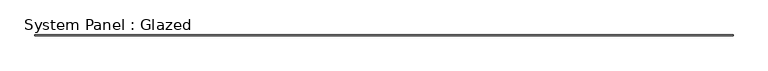
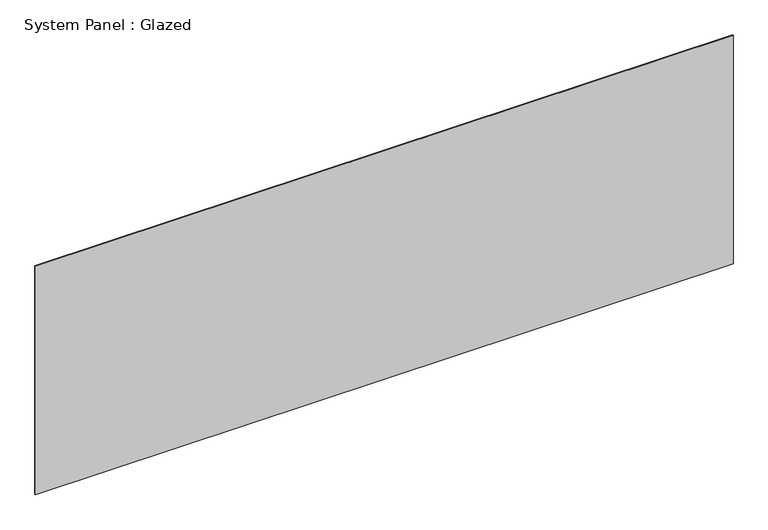
"""IFC4 building model written with IfcOpenShell, lengths in millimetres: plate geometry, System Panel : Glazed."""

import ifcopenshell
import ifcopenshell.guid

model = None  # the IFC model being written
_history = None  # IfcOwnerHistory: only IFC2X3 demands one
_inside = {}  # id of a spatial element -> (the spatial element, [elements in it])
_under = {}  # id of a project, library or spatial element -> (it, [spatial elements below it])
_declared = {}  # id of a project -> (the project, [libraries it declares])
_typed = {}  # id of a type object -> (the type object, [elements of that type])
_made_of = {}  # id of a material, layer set ... -> (it, [elements and type objects made of it])


def new_model(schema):
    """Start an empty IFC model of exactly this schema.

    Asked for "IFC4X3", IfcOpenShell would pick the latest addendum, in which some entities
    have other attributes; the version numbers below select the first issue.
    IFC2X3 requires an IfcOwnerHistory on every rooted entity: one is made here for all.
    """
    global model, _history
    if schema == "IFC4X3":
        model = ifcopenshell.file(schema_version=(4, 3, 0, 0))
    else:
        model = ifcopenshell.file(schema=schema)
    _inside.clear()
    _under.clear()
    _declared.clear()
    _typed.clear()
    _made_of.clear()
    _history = None
    if model.schema == "IFC2X3":
        org = make("IfcOrganization", Name="unknown")
        user = make(
            "IfcPersonAndOrganization",
            ThePerson=make("IfcPerson", FamilyName="unknown"),
            TheOrganization=org,
        )
        app = make(
            "IfcApplication",
            ApplicationDeveloper=org,
            Version="unknown",
            ApplicationFullName="unknown",
            ApplicationIdentifier="unknown",
        )
        _history = make(
            "IfcOwnerHistory",
            OwningUser=user,
            OwningApplication=app,
            ChangeAction="ADDED",
            CreationDate=0,
        )
    return model


def make(cls, **values):
    """One entity of the class cls with the attributes given. An attribute that is None is left unset."""
    return model.create_entity(
        cls, **{name: value for name, value in values.items() if value is not None}
    )


def rooted(cls, **values):
    """An entity with a GlobalId (a new one), such as an element, a storey or a relation."""
    return make(cls, GlobalId=ifcopenshell.guid.new(), OwnerHistory=_history, **values)


def si_unit(unit_type, name, prefix=None):
    """IfcSIUnit, for example si_unit("LENGTHUNIT", "METRE", prefix="MILLI")."""
    return make("IfcSIUnit", UnitType=unit_type, Prefix=prefix, Name=name)


def assignment(units):
    """IfcUnitAssignment: the units of a project."""
    return None if units is None else make("IfcUnitAssignment", Units=units)


def point(xyz):
    """IfcCartesianPoint."""
    return None if xyz is None else make("IfcCartesianPoint", Coordinates=xyz)


def direction(xyz):
    """IfcDirection."""
    return None if xyz is None else make("IfcDirection", DirectionRatios=xyz)


def frame(location, z_axis=None, x_axis=None):
    """IfcAxis2Placement3D, a coordinate frame: its origin and axes. An axis left out is left unset."""
    return make(
        "IfcAxis2Placement3D",
        Location=point(location),
        Axis=direction(z_axis),
        RefDirection=direction(x_axis),
    )


def origin():
    """The frame at (0, 0, 0) with its axes left unset."""
    return frame((0.0, 0.0, 0.0))


def origin_with_axes():
    """The frame at (0, 0, 0) with the z axis (0, 0, 1) and the x axis (1, 0, 0) written out."""
    return frame((0.0, 0.0, 0.0), z_axis=(0.0, 0.0, 1.0), x_axis=(1.0, 0.0, 0.0))


def place(relative_to, where):
    """IfcLocalPlacement: puts the frame where relative to a parent placement (None: the world)."""
    return make(
        "IfcLocalPlacement", PlacementRelTo=relative_to, RelativePlacement=where
    )


def context(
    kind, dimensions, precision=None, world=None, true_north=None, identifier=None
):
    """IfcGeometricRepresentationContext, for example the 3D "Model" context."""
    return make(
        "IfcGeometricRepresentationContext",
        ContextIdentifier=identifier,
        ContextType=kind,
        CoordinateSpaceDimension=dimensions,
        Precision=precision,
        WorldCoordinateSystem=world,
        TrueNorth=true_north,
    )


def project(units=None, contexts=None):
    """IfcProject with its units and contexts."""
    return rooted(
        "IfcProject",
        Name="project",
        RepresentationContexts=contexts,
        UnitsInContext=assignment(units),
    )


def spatial(cls, under=None, at=None, **own):
    """A site, building, storey or space (cls), placed at a placement, below another one or the project."""
    s = rooted(cls, ObjectPlacement=at, **own)
    if under is not None:
        _under.setdefault(under.id(), (under, []))[1].append(s)
    return s


def polyline(points):
    """IfcPolyline through the points."""
    return make("IfcPolyline", Points=[point(p) for p in points])


def outline(outer, holes=None, kind="AREA"):
    """IfcArbitraryClosedProfileDef: a profile drawn as a closed curve; with holes, ...WithVoids."""
    if holes is None:
        return make("IfcArbitraryClosedProfileDef", ProfileType=kind, OuterCurve=outer)
    return make(
        "IfcArbitraryProfileDefWithVoids",
        ProfileType=kind,
        OuterCurve=outer,
        InnerCurves=holes,
    )


def extrude(swept, where, along, depth):
    """IfcExtrudedAreaSolid: the profile swept, set in the frame where, extruded along a direction by depth."""
    return make(
        "IfcExtrudedAreaSolid",
        SweptArea=swept,
        Position=where,
        ExtrudedDirection=direction(along),
        Depth=depth,
    )


def shape(context_of_items, identifier, shape_type, items):
    """IfcShapeRepresentation: the items that make up one representation, for example the "Body"."""
    return make(
        "IfcShapeRepresentation",
        ContextOfItems=context_of_items,
        RepresentationIdentifier=identifier,
        RepresentationType=shape_type,
        Items=items,
    )


def source(mapping_origin, context_of_items, identifier, shape_type, items):
    """IfcRepresentationMap: a shape defined once, which mapped items show again and again."""
    return make(
        "IfcRepresentationMap",
        MappingOrigin=mapping_origin,
        MappedRepresentation=shape(context_of_items, identifier, shape_type, items),
    )


def transform(
    local_origin,
    x_axis=None,
    y_axis=None,
    z_axis=None,
    scale=None,
    scale2=None,
    scale3=None,
    uniform=True,
):
    """IfcCartesianTransformationOperator3D, or its non-uniform kind. x_axis, y_axis, z_axis: its Axis1, 2, 3."""
    if uniform:
        return make(
            "IfcCartesianTransformationOperator3D",
            Axis1=direction(x_axis),
            Axis2=direction(y_axis),
            LocalOrigin=point(local_origin),
            Scale=scale,
            Axis3=direction(z_axis),
        )
    return make(
        "IfcCartesianTransformationOperator3DnonUniform",
        Axis1=direction(x_axis),
        Axis2=direction(y_axis),
        LocalOrigin=point(local_origin),
        Scale=scale,
        Axis3=direction(z_axis),
        Scale2=scale2,
        Scale3=scale3,
    )


def mapped(mapping_source, mapping_target):
    """IfcMappedItem: shows the shape of a source again, moved by a transform."""
    return make(
        "IfcMappedItem", MappingSource=mapping_source, MappingTarget=mapping_target
    )


def made_of(thing, what):
    """Note that an element or type object is made of a material, layer set ...; save() writes the relation."""
    if what is not None:
        _made_of.setdefault(what.id(), (what, []))[1].append(thing)
    return thing


def element(
    cls,
    number,
    at=None,
    inside=None,
    cuts=None,
    type_object=None,
    material=None,
    context=None,
    identifier="Body",
    shape_type=None,
    held_by="IfcProductDefinitionShape",
    body=None,
    shapes=None,
    **own,
):
    """One element of the class cls, such as IfcWall. Its Tag is "e" and its number.

    at: its placement. inside: the storey or other place that contains it. cuts: it is an
    opening in that element (IfcRelVoidsElement). A single representation is given by context,
    identifier, shape_type and body (its items); several are given by shapes. held_by: the class
    of the entity that holds the representations. save() writes the other relations.
    """
    e = rooted(cls, Tag="e%d" % number, ObjectPlacement=at, **own)
    if body is not None:
        shapes = [shape(context, identifier, shape_type, body)]
    if shapes is not None:
        e.Representation = make(held_by, Representations=shapes)
    if inside is not None:
        _inside.setdefault(inside.id(), (inside, []))[1].append(e)
    if cuts is not None:
        rooted(
            "IfcRelVoidsElement", RelatingBuildingElement=cuts, RelatedOpeningElement=e
        )
    if type_object is not None:
        _typed.setdefault(type_object.id(), (type_object, []))[1].append(e)
    return made_of(e, material)


def aggregate(whole, parts):
    """IfcRelAggregates: a whole, such as a stair, and the parts it consists of."""
    return rooted("IfcRelAggregates", RelatingObject=whole, RelatedObjects=parts)


def save(model, path):
    """Write the relations noted so far, then the file.

    IfcRelAggregates (storeys below a building ...), IfcRelContainedInSpatialStructure (elements
    in a storey), IfcRelDefinesByType, IfcRelAssociatesMaterial and IfcRelDeclares: one each for
    every whole, place, type object, material and project.
    """
    for whole, parts in _under.values():
        aggregate(whole, parts)
    for where, things in _inside.values():
        rooted(
            "IfcRelContainedInSpatialStructure",
            RelatedElements=things,
            RelatingStructure=where,
        )
    for kind, things in _typed.values():
        rooted("IfcRelDefinesByType", RelatedObjects=things, RelatingType=kind)
    for what, things in _made_of.values():
        rooted("IfcRelAssociatesMaterial", RelatedObjects=things, RelatingMaterial=what)
    for by, libraries in _declared.values():
        rooted("IfcRelDeclares", RelatingContext=by, RelatedDefinitions=libraries)
    model.write(path)


def system_panel_glazed_8cf960c6(model_context):
    return source(origin(), model_context, "Body", "SweptSolid", [
        extrude(outline(polyline([(13000.0, 24.5), (-13000.0, 24.5), (-13000.0, 49.5), (13000.0, 49.5), (13000.0, 24.5)])), origin_with_axes(), (0.0, 0.0, 1.0), 9000.0),
    ])


if __name__ == "__main__":
    model = new_model("IFC4")
    model_context = context("Model", 3, world=origin())
    ifc_project = project(units=[si_unit("LENGTHUNIT", "METRE", prefix="MILLI")], contexts=[model_context])
    site = spatial("IfcSite", under=ifc_project)
    building = spatial("IfcBuilding", under=site)
    placement = place(None, origin())
    system_panel_glazed_shape = system_panel_glazed_8cf960c6(model_context)
    element("IfcPlate", 1, ObjectType="System Panel : Glazed", at=placement, inside=building, context=model_context, shape_type="MappedRepresentation", body=[
        mapped(system_panel_glazed_shape, transform((0.0, 0.0, 0.0), x_axis=(1.0, 0.0, 0.0), y_axis=(0.0, 1.0, 0.0), z_axis=(0.0, 0.0, 1.0))),
    ])
    save(model, "model.ifc")

# Revit data of these elements
# Element 1 (IfcPlate, "System Panel : Glazed")
#   Materials on its faces: "Glass"
# Materials
#   "Glass": class "Glass", colour RGB 0 128 192, transparency 0.9
